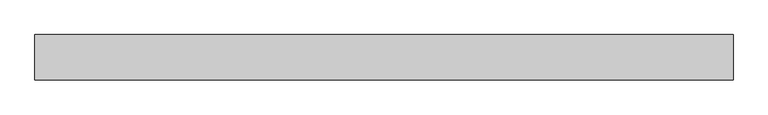
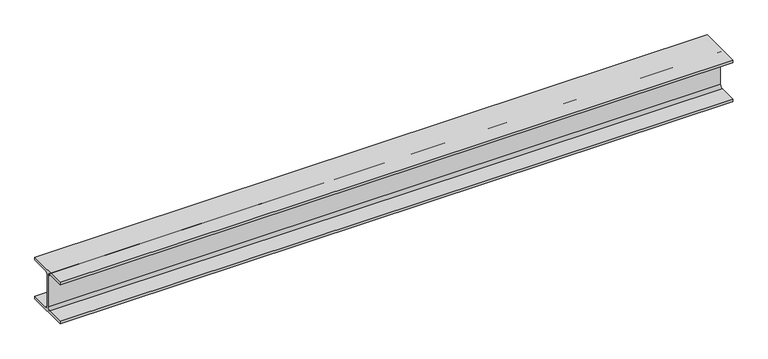
"""IFC4 building model written with IfcOpenShell, lengths in millimetres: beam geometry, 0912_Steel Framing_H-KSD3502 : H_SB_ASB_H-200x200x8x12."""

from ifc_helpers import new_model, si_unit, point, frame, frame_2d, origin, place, context, project, spatial, polyline, circle_curve, trimmed, segment, composite_curve, outline, extrude, source, transform, mapped, element, save


def beam_1885582d(model_context):
    return source(origin(), model_context, "Body", "SweptSolid", [
        extrude(outline(composite_curve([segment(polyline([(100.0, -88.0), (100.0, -100.0), (-100.0, -100.0), (-100.0, -88.0), (-17.0, -88.0)]), True, "CONTINUOUS"), segment(trimmed(circle_curve(frame_2d((-17.0, -75.0)), 13.0), [point((-17.0, -88.0))], [point((-4.0, -75.0))], True, "CARTESIAN"), True, "CONTINUOUS"), segment(polyline([(-4.0, -75.0), (-4.0, 75.0)]), True, "CONTINUOUS"), segment(trimmed(circle_curve(frame_2d((-17.0, 75.0)), 13.0), [point((-4.0, 75.0))], [point((-17.0, 88.0))], True, "CARTESIAN"), True, "CONTINUOUS"), segment(polyline([(-17.0, 88.0), (-100.0, 88.0), (-100.0, 100.0), (100.0, 100.0), (100.0, 88.0), (17.0, 88.0)]), True, "CONTINUOUS"), segment(trimmed(circle_curve(frame_2d((17.0, 75.0)), 13.0), [point((17.0, 88.0))], [point((4.0, 75.0))], True, "CARTESIAN"), True, "CONTINUOUS"), segment(polyline([(4.0, 75.0), (4.0, -75.0)]), True, "CONTINUOUS"), segment(trimmed(circle_curve(frame_2d((17.0, -75.0)), 13.0), [point((4.0, -75.0))], [point((17.0, -88.0))], True, "CARTESIAN"), True, "CONTINUOUS"), segment(polyline([(17.0, -88.0), (100.0, -88.0)]), True, "CONTINUOUS")], self_intersect=False)), frame((-1489.1986147, 0.0, 0.0), z_axis=(1.0, 0.0, 0.0), x_axis=(0.0, 1.0, 0.0)), (0.0, 0.0, 1.0), 3067.173634),
    ])


if __name__ == "__main__":
    model = new_model("IFC4")
    model_context = context("Model", 3, world=origin())
    ifc_project = project(units=[si_unit("LENGTHUNIT", "METRE", prefix="MILLI")], contexts=[model_context])
    site = spatial("IfcSite", under=ifc_project)
    building = spatial("IfcBuilding", under=site)
    placement = place(None, origin())
    beam_shape = beam_1885582d(model_context)
    element("IfcBeam", 1, ObjectType="0912_Steel Framing_H-KSD3502 : H_SB_ASB_H-200x200x8x12", at=placement, inside=building, context=model_context, shape_type="MappedRepresentation", body=[
        mapped(beam_shape, transform((0.0, 0.0, 0.0), x_axis=(1.0, 0.0, 0.0), y_axis=(0.0, 1.0, 0.0), z_axis=(0.0, 0.0, 1.0))),
    ])
    save(model, "model.ifc")

# Revit data of these elements
# Type "0912_Steel Framing_H-KSD3502 : H_SB_ASB_H-200x200x8x12"
#   H_WM Code_1 = "S01AA002-00001 | Main Steel Structure Fabrication Work | Shelter/Building | Medium Steel - Standard (90KG/M>Weight≥30KG/M) | Material: (   )"
#   H_WM Code_2 = "S03AA028-00001 | Main Steel Structure Erection Work | Shelter/Building | Medium Steel (90KG/M>Weight≥30KG/M) | Material: (   )"
#   H_WM Code_3 = "S01AA010-00001 | Main Steel Structure Fabrication Work | Shelter/Building | Steel Painting/Coating | for Non-Fireproofed Steel Surface, Surface Preparation, Primer, Second & Final Coat | Material: (   )"
#   H_Q'ty Cal Type Tag = "SB-Q2"
#   Width = 20.0 cm
#   Web Thickness = 0.8 cm
#   Web Fillet = 1.3 cm
#   Warping Constant = 141000.0 cm⁶
#   W = 0
#   Torsional Moment of Inertia = 26.2485 cm⁴
#   Section Area = 63.53 cm²
#   Plastic Modulus weak axis = 244.0 cm³
#   Plastic Modulus strong axis = 525.0 cm³
#   Perimeter = 1.16 m²/m
#   Nominal Weight = 49.90 kgf/m
#   Moment of Inertia weak axis = 1600.00 cm⁴
#   Moment of Inertia strong axis = 4720.00 cm⁴
#   Height = 20.0 cm
#   Flange Thickness = 1.2 cm
#   Elastic Modulus weak axis = 160.0 cm³
#   Elastic Modulus strong axis = 472.0 cm³
#   Centroid Vertical = 10.0 cm
#   Centroid Horizontal = 10.0 cm
#   Ix = 47200000
#   Length [instance default] = 1.5240 m
#   Zx = 525000
#   b = 0.2000 m
#   h = 0.2000 m
#   r = 0.0130 m
#   s = 0.0080 m
#   t = 0.0120 m
#   A = 0.006353 m²
#   Structural Material [instance default] = Steel, 45-345
#   Assembly Code = ""
# Element 1 (IfcBeam, "0912_Steel Framing_H-KSD3502 : H_SB_ASB_H-200x200x8x12")
#   Structural Material = none
# Materials
#   "Steel, 45-345": class "Metal", colour RGB 189 187 185, transparency 0, Description = "Steel 345 MPa", Cost = 0
